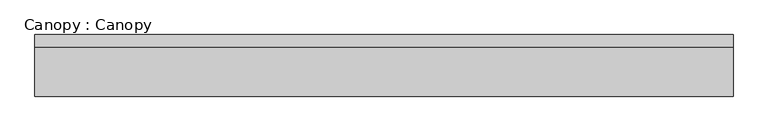
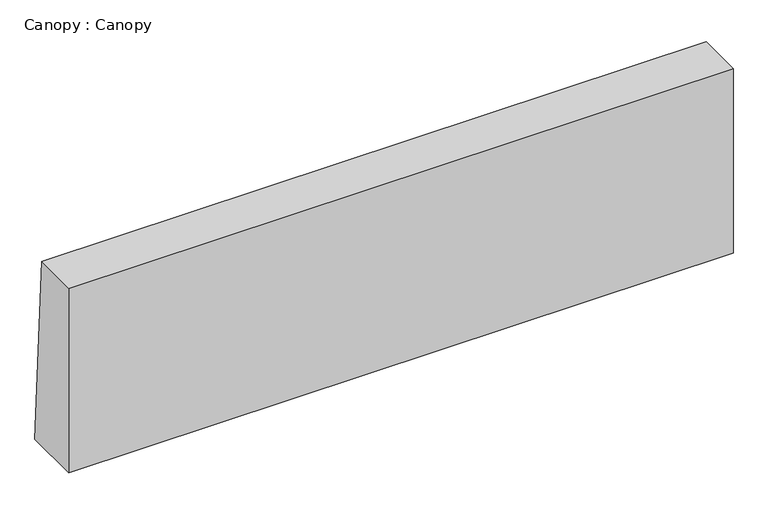
"""IFC4 building model written with IfcOpenShell, lengths in millimetres: proxy geometry, Canopy : Canopy."""

from ifc_helpers import new_model, si_unit, frame, origin, place, context, project, spatial, polyline, outline, extrude, source, transform, mapped, element, save


def canopy_canopy_9389d072(model_context):
    return source(origin(), model_context, "Body", "SweptSolid", [
        extrude(outline(polyline([(150.0, 0.0), (0.0, 0.0), (0.0, 500.0), (120.0, 500.0), (150.0, 0.0)])), frame((-850.0, 0.0, 0.0), z_axis=(1.0, 0.0, 0.0), x_axis=(0.0, 1.0, 0.0)), (0.0, 0.0, 1.0), 1700.0),
    ])


if __name__ == "__main__":
    model = new_model("IFC4")
    model_context = context("Model", 3, world=origin())
    ifc_project = project(units=[si_unit("LENGTHUNIT", "METRE", prefix="MILLI")], contexts=[model_context])
    site = spatial("IfcSite", under=ifc_project)
    building = spatial("IfcBuilding", under=site)
    placement = place(None, origin())
    canopy_canopy_shape = canopy_canopy_9389d072(model_context)
    element("IfcBuildingElementProxy", 1, Name="Canopy : Canopy", ObjectType="Canopy : Canopy", at=placement, inside=building, context=model_context, shape_type="MappedRepresentation", body=[
        mapped(canopy_canopy_shape, transform((0.0, 0.0, 0.0), x_axis=(1.0, 0.0, 0.0), y_axis=(0.0, 1.0, 0.0), z_axis=(0.0, 0.0, 1.0))),
    ])
    save(model, "model.ifc")

# Revit data of these elements
# Type "Canopy : Canopy"
#   Type Comments = "CV-AG"
#   H_Rebar Ratio = 0.1
#   Canopy Width [instance default] = 1700 mm
#   Canopy Length [instance default] = 1000 mm
#   Canopy L.P = 120 mm
#   Canopy H.P = 150 mm
#   구조재료 = Concrete_f'c=28MPa(Cylender)
#   Default Elevation = 0
# Element 1 (IfcBuildingElementProxy, "Canopy : Canopy")
#   Canopy Length = 500 mm
#   Materials on its faces: "Concrete_f'c=28MPa(Cylender)"
# Materials
#   "Concrete_f'c=28MPa(Cylender)": class "Concrete", colour RGB 176 176 176, transparency 0, Description = "Reinf. Conc.", Cost = 0, Image = Concrete.Cast-In-Place.Flat.Polished.Grey.jpg
